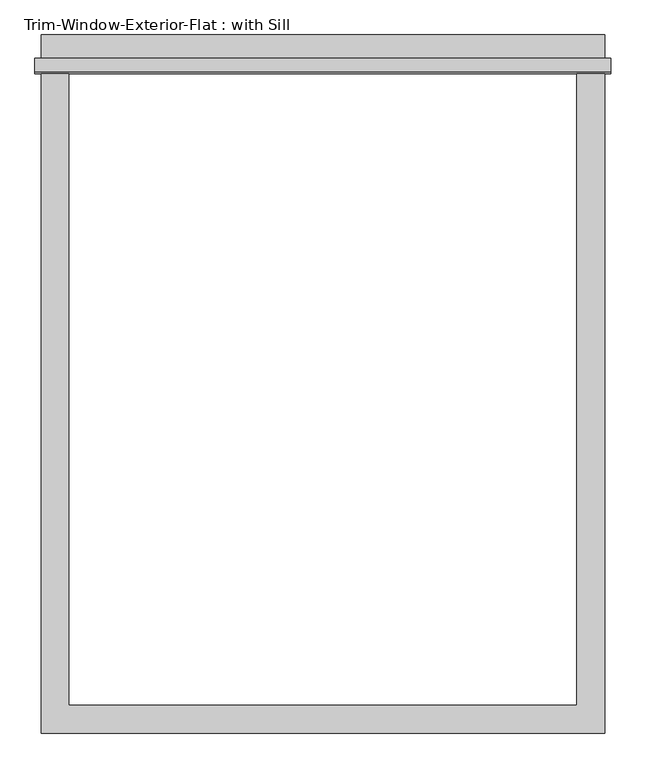
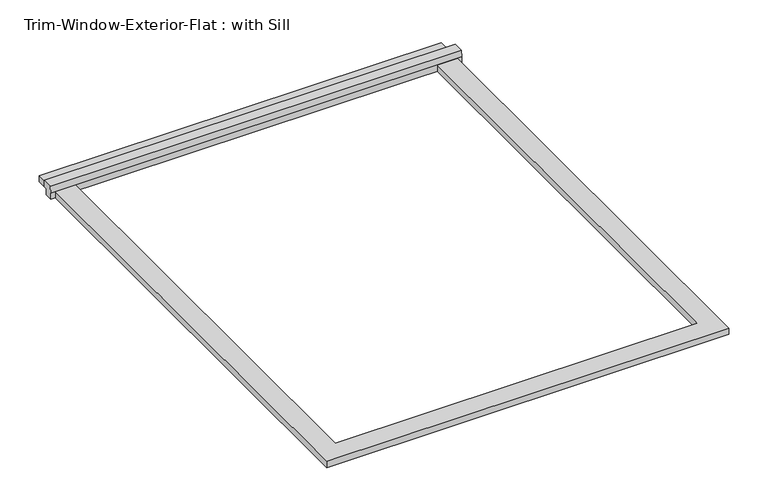
"""IFC4 building model written with IfcOpenShell, lengths in millimetres: proxy geometry, Trim-Window-Exterior-Flat : with Sill."""

from ifc_helpers import new_model, si_unit, frame, origin, origin_with_axes, place, context, project, spatial, polyline, outline, extrude, source, transform, mapped, element, save


def trim_window_exterior_flat_with_sill_7ce58be9(model_context):
    return source(origin(), model_context, "Body", "SweptSolid", [
        extrude(outline(polyline([(577.85, 1317.5823709), (-577.85, 1317.5823709), (-577.85, 1374.7323709), (577.85, 1374.7323709), (577.85, 1317.5823709)])), origin_with_axes(), (0.0, 0.0, 1.0), 19.05),
        extrude(outline(polyline([(1327.15, 38.1), (1327.15, 19.05), (1317.5823709, 19.05), (1317.5823709, 0.0), (1295.4, 0.0), (1295.4, 19.05), (1297.8580645, 38.1), (1327.15, 38.1)])), frame((-590.55, 0.0, 0.0), z_axis=(1.0, 0.0, 0.0), x_axis=(0.0, 1.0, 0.0)), (0.0, 0.0, 1.0), 1181.1),
        extrude(outline(polyline([(-577.85, -57.15), (-577.85, 1295.4), (-520.7, 1295.4), (-520.7, 0.0), (520.7, 0.0), (520.7, 1295.4), (577.85, 1295.4), (577.85, -57.15), (-577.85, -57.15)])), origin_with_axes(), (0.0, 0.0, 1.0), 19.05),
    ])


if __name__ == "__main__":
    model = new_model("IFC4")
    model_context = context("Model", 3, world=origin())
    ifc_project = project(units=[si_unit("LENGTHUNIT", "METRE", prefix="MILLI")], contexts=[model_context])
    site = spatial("IfcSite", under=ifc_project)
    building = spatial("IfcBuilding", under=site)
    placement = place(None, origin())
    trim_window_exterior_flat_with_sill_shape = trim_window_exterior_flat_with_sill_7ce58be9(model_context)
    element("IfcBuildingElementProxy", 1, Name="Trim-Window-Exterior-Flat : with Sill", ObjectType="Trim-Window-Exterior-Flat : with Sill", at=placement, inside=building, context=model_context, shape_type="MappedRepresentation", body=[
        mapped(trim_window_exterior_flat_with_sill_shape, transform((0.0, 0.0, 0.0), x_axis=(1.0, 0.0, 0.0), y_axis=(0.0, 1.0, 0.0), z_axis=(0.0, 0.0, 1.0))),
    ])
    save(model, "model.ifc")

# Revit data of these elements
# Type "Trim-Window-Exterior-Flat : with Sill"
#   Trim Width = 0' - 2 1/4"
#   Trim Thickness_Picture Frame = 0' - 1 1/4"
#   Trim Thickness_with Sill = 0' - 0 3/4"
#   Sill Thickness = 0' - 1 1/4"
#   Opening Width [instance default] = 2' - 0"
#   Opening Height [instance default] = 3' - 0"
#   Default Elevation = 4' - 0"
#   Sill = yes
#   Picture Frame = no
#   Trim Material [instance default] = none
# Element 1 (IfcBuildingElementProxy, "Trim-Window-Exterior-Flat : with Sill")
#   Opening Width = 3' - 5"
#   Opening Height = 4' - 3"
#   Trim Material = Clad - White
#   Materials on its faces: "Clad - White"
# Materials
#   "Clad - White": class "Wood", colour RGB 242 242 238, transparency 0, Cost = 0
